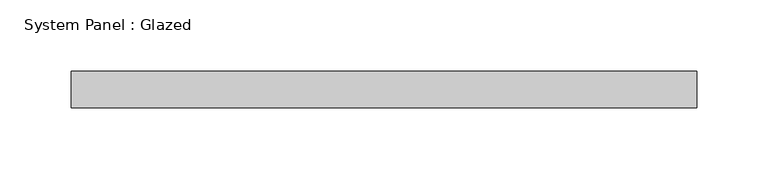
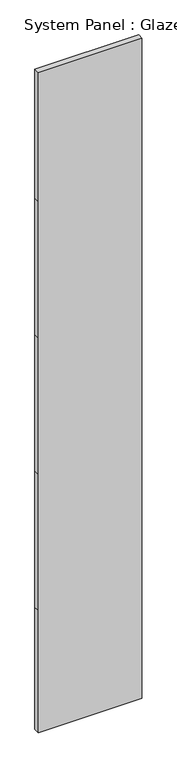
"""IFC4 building model written with IfcOpenShell, lengths in millimetres: plate geometry, System Panel : Glazed."""

from ifc_helpers import new_model, si_unit, frame, origin, place, context, project, spatial, polyline, outline, extrude, source, transform, mapped, element, save


def system_panel_glazed_6ebbee62(model_context):
    return source(origin(), model_context, "Body", "SweptSolid", [
        extrude(outline(polyline([(0.0, -219.075), (0.0, 219.075), (546.1, 219.075), (1155.7, 219.075), (1765.3, 219.075), (2374.9, 219.075), (2952.75, 219.075), (2952.75, -219.075), (2374.9, -219.075), (1765.3, -219.075), (1155.7, -219.075), (546.1, -219.075), (0.0, -219.075)])), frame((0.0, -44.45, 0.0), z_axis=(0.0, 1.0, 0.0), x_axis=(0.0, 0.0, 1.0)), (0.0, 0.0, 1.0), 25.4),
    ])


if __name__ == "__main__":
    model = new_model("IFC4")
    model_context = context("Model", 3, world=origin())
    ifc_project = project(units=[si_unit("LENGTHUNIT", "METRE", prefix="MILLI")], contexts=[model_context])
    site = spatial("IfcSite", under=ifc_project)
    building = spatial("IfcBuilding", under=site)
    placement = place(None, origin())
    system_panel_glazed_shape = system_panel_glazed_6ebbee62(model_context)
    element("IfcPlate", 1, ObjectType="System Panel : Glazed", at=placement, inside=building, context=model_context, shape_type="MappedRepresentation", body=[
        mapped(system_panel_glazed_shape, transform((0.0, 0.0, 0.0), x_axis=(1.0, 0.0, 0.0), y_axis=(0.0, 1.0, 0.0), z_axis=(0.0, 0.0, 1.0))),
    ])
    save(model, "model.ifc")

# Revit data of these elements
# Element 1 (IfcPlate, "System Panel : Glazed")
#   Materials on its faces: "Glass"
# Materials
#   "Glass": class "Unassigned", colour RGB 147 173 200, transparency 0.7, Cost = 0
